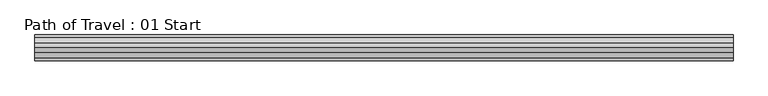
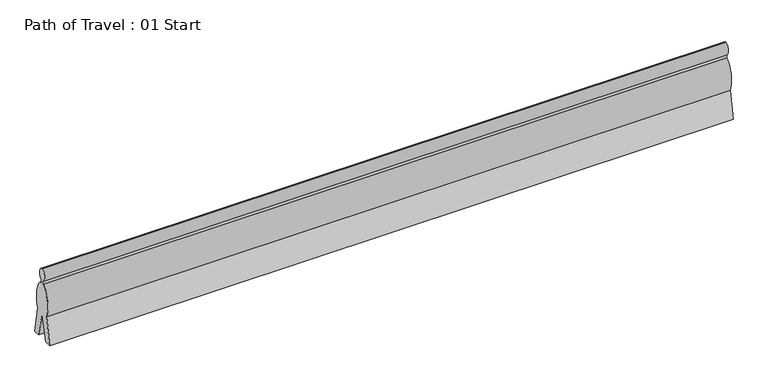
"""IFC4 building model written with IfcOpenShell, lengths in millimetres: proxy geometry, Path of Travel : 01 Start."""

import ifcopenshell
import ifcopenshell.guid

model = None  # the IFC model being written
_history = None  # IfcOwnerHistory: only IFC2X3 demands one
_inside = {}  # id of a spatial element -> (the spatial element, [elements in it])
_under = {}  # id of a project, library or spatial element -> (it, [spatial elements below it])
_declared = {}  # id of a project -> (the project, [libraries it declares])
_typed = {}  # id of a type object -> (the type object, [elements of that type])
_made_of = {}  # id of a material, layer set ... -> (it, [elements and type objects made of it])


def new_model(schema):
    """Start an empty IFC model of exactly this schema.

    Asked for "IFC4X3", IfcOpenShell would pick the latest addendum, in which some entities
    have other attributes; the version numbers below select the first issue.
    IFC2X3 requires an IfcOwnerHistory on every rooted entity: one is made here for all.
    """
    global model, _history
    if schema == "IFC4X3":
        model = ifcopenshell.file(schema_version=(4, 3, 0, 0))
    else:
        model = ifcopenshell.file(schema=schema)
    _inside.clear()
    _under.clear()
    _declared.clear()
    _typed.clear()
    _made_of.clear()
    _history = None
    if model.schema == "IFC2X3":
        org = make("IfcOrganization", Name="unknown")
        user = make(
            "IfcPersonAndOrganization",
            ThePerson=make("IfcPerson", FamilyName="unknown"),
            TheOrganization=org,
        )
        app = make(
            "IfcApplication",
            ApplicationDeveloper=org,
            Version="unknown",
            ApplicationFullName="unknown",
            ApplicationIdentifier="unknown",
        )
        _history = make(
            "IfcOwnerHistory",
            OwningUser=user,
            OwningApplication=app,
            ChangeAction="ADDED",
            CreationDate=0,
        )
    return model


def make(cls, **values):
    """One entity of the class cls with the attributes given. An attribute that is None is left unset."""
    return model.create_entity(
        cls, **{name: value for name, value in values.items() if value is not None}
    )


def rooted(cls, **values):
    """An entity with a GlobalId (a new one), such as an element, a storey or a relation."""
    return make(cls, GlobalId=ifcopenshell.guid.new(), OwnerHistory=_history, **values)


def si_unit(unit_type, name, prefix=None):
    """IfcSIUnit, for example si_unit("LENGTHUNIT", "METRE", prefix="MILLI")."""
    return make("IfcSIUnit", UnitType=unit_type, Prefix=prefix, Name=name)


def assignment(units):
    """IfcUnitAssignment: the units of a project."""
    return None if units is None else make("IfcUnitAssignment", Units=units)


def point(xyz):
    """IfcCartesianPoint."""
    return None if xyz is None else make("IfcCartesianPoint", Coordinates=xyz)


def direction(xyz):
    """IfcDirection."""
    return None if xyz is None else make("IfcDirection", DirectionRatios=xyz)


def frame(location, z_axis=None, x_axis=None):
    """IfcAxis2Placement3D, a coordinate frame: its origin and axes. An axis left out is left unset."""
    return make(
        "IfcAxis2Placement3D",
        Location=point(location),
        Axis=direction(z_axis),
        RefDirection=direction(x_axis),
    )


def origin():
    """The frame at (0, 0, 0) with its axes left unset."""
    return frame((0.0, 0.0, 0.0))


def place(relative_to, where):
    """IfcLocalPlacement: puts the frame where relative to a parent placement (None: the world)."""
    return make(
        "IfcLocalPlacement", PlacementRelTo=relative_to, RelativePlacement=where
    )


def context(
    kind, dimensions, precision=None, world=None, true_north=None, identifier=None
):
    """IfcGeometricRepresentationContext, for example the 3D "Model" context."""
    return make(
        "IfcGeometricRepresentationContext",
        ContextIdentifier=identifier,
        ContextType=kind,
        CoordinateSpaceDimension=dimensions,
        Precision=precision,
        WorldCoordinateSystem=world,
        TrueNorth=true_north,
    )


def project(units=None, contexts=None):
    """IfcProject with its units and contexts."""
    return rooted(
        "IfcProject",
        Name="project",
        RepresentationContexts=contexts,
        UnitsInContext=assignment(units),
    )


def spatial(cls, under=None, at=None, **own):
    """A site, building, storey or space (cls), placed at a placement, below another one or the project."""
    s = rooted(cls, ObjectPlacement=at, **own)
    if under is not None:
        _under.setdefault(under.id(), (under, []))[1].append(s)
    return s


def ellipse_curve(where, semi_axis1, semi_axis2):
    """IfcEllipse in the frame where."""
    return make(
        "IfcEllipse", Position=where, SemiAxis1=semi_axis1, SemiAxis2=semi_axis2
    )


def trimmed(basis, trim1, trim2, sense, master):
    """IfcTrimmedCurve: the piece of a basis curve between two trims."""
    return make(
        "IfcTrimmedCurve",
        BasisCurve=basis,
        Trim1=trim1,
        Trim2=trim2,
        SenseAgreement=sense,
        MasterRepresentation=master,
    )


def shape(context_of_items, identifier, shape_type, items):
    """IfcShapeRepresentation: the items that make up one representation, for example the "Body"."""
    return make(
        "IfcShapeRepresentation",
        ContextOfItems=context_of_items,
        RepresentationIdentifier=identifier,
        RepresentationType=shape_type,
        Items=items,
    )


def source(mapping_origin, context_of_items, identifier, shape_type, items):
    """IfcRepresentationMap: a shape defined once, which mapped items show again and again."""
    return make(
        "IfcRepresentationMap",
        MappingOrigin=mapping_origin,
        MappedRepresentation=shape(context_of_items, identifier, shape_type, items),
    )


def transform(
    local_origin,
    x_axis=None,
    y_axis=None,
    z_axis=None,
    scale=None,
    scale2=None,
    scale3=None,
    uniform=True,
):
    """IfcCartesianTransformationOperator3D, or its non-uniform kind. x_axis, y_axis, z_axis: its Axis1, 2, 3."""
    if uniform:
        return make(
            "IfcCartesianTransformationOperator3D",
            Axis1=direction(x_axis),
            Axis2=direction(y_axis),
            LocalOrigin=point(local_origin),
            Scale=scale,
            Axis3=direction(z_axis),
        )
    return make(
        "IfcCartesianTransformationOperator3DnonUniform",
        Axis1=direction(x_axis),
        Axis2=direction(y_axis),
        LocalOrigin=point(local_origin),
        Scale=scale,
        Axis3=direction(z_axis),
        Scale2=scale2,
        Scale3=scale3,
    )


def mapped(mapping_source, mapping_target):
    """IfcMappedItem: shows the shape of a source again, moved by a transform."""
    return make(
        "IfcMappedItem", MappingSource=mapping_source, MappingTarget=mapping_target
    )


def made_of(thing, what):
    """Note that an element or type object is made of a material, layer set ...; save() writes the relation."""
    if what is not None:
        _made_of.setdefault(what.id(), (what, []))[1].append(thing)
    return thing


def element(
    cls,
    number,
    at=None,
    inside=None,
    cuts=None,
    type_object=None,
    material=None,
    context=None,
    identifier="Body",
    shape_type=None,
    held_by="IfcProductDefinitionShape",
    body=None,
    shapes=None,
    **own,
):
    """One element of the class cls, such as IfcWall. Its Tag is "e" and its number.

    at: its placement. inside: the storey or other place that contains it. cuts: it is an
    opening in that element (IfcRelVoidsElement). A single representation is given by context,
    identifier, shape_type and body (its items); several are given by shapes. held_by: the class
    of the entity that holds the representations. save() writes the other relations.
    """
    e = rooted(cls, Tag="e%d" % number, ObjectPlacement=at, **own)
    if body is not None:
        shapes = [shape(context, identifier, shape_type, body)]
    if shapes is not None:
        e.Representation = make(held_by, Representations=shapes)
    if inside is not None:
        _inside.setdefault(inside.id(), (inside, []))[1].append(e)
    if cuts is not None:
        rooted(
            "IfcRelVoidsElement", RelatingBuildingElement=cuts, RelatedOpeningElement=e
        )
    if type_object is not None:
        _typed.setdefault(type_object.id(), (type_object, []))[1].append(e)
    return made_of(e, material)


def aggregate(whole, parts):
    """IfcRelAggregates: a whole, such as a stair, and the parts it consists of."""
    return rooted("IfcRelAggregates", RelatingObject=whole, RelatedObjects=parts)


def save(model, path):
    """Write the relations noted so far, then the file.

    IfcRelAggregates (storeys below a building ...), IfcRelContainedInSpatialStructure (elements
    in a storey), IfcRelDefinesByType, IfcRelAssociatesMaterial and IfcRelDeclares: one each for
    every whole, place, type object, material and project.
    """
    for whole, parts in _under.values():
        aggregate(whole, parts)
    for where, things in _inside.values():
        rooted(
            "IfcRelContainedInSpatialStructure",
            RelatedElements=things,
            RelatingStructure=where,
        )
    for kind, things in _typed.values():
        rooted("IfcRelDefinesByType", RelatedObjects=things, RelatingType=kind)
    for what, things in _made_of.values():
        rooted("IfcRelAssociatesMaterial", RelatedObjects=things, RelatingMaterial=what)
    for by, libraries in _declared.values():
        rooted("IfcRelDeclares", RelatingContext=by, RelatedDefinitions=libraries)
    model.write(path)


def plane_surface(at):
    """IfcPlane: the flat surface through the origin of the frame at, square to its z axis."""
    return make("IfcPlane", Position=at)


def extruded_surface(curve, direction_of_extrusion, depth):
    """IfcSurfaceOfLinearExtrusion: the curve pushed along a direction by depth."""
    return make(
        "IfcSurfaceOfLinearExtrusion",
        SweptCurve=make("IfcArbitraryOpenProfileDef", ProfileType="CURVE", Curve=curve),
        ExtrudedDirection=direction(direction_of_extrusion),
        Depth=depth,
    )


def advanced_brep(points, edges, surfaces, faces):
    """IfcAdvancedBrep: a solid bounded by faces that lie on surfaces and meet in shared edges.

    An edge is (start, end): straight between two places in points (the first is 0);
    or (start, end, curve); or (start, end, curve, False) where it runs against its curve.
    A face is (place in surfaces, loops), or (place, loops, False) where it looks against
    its surface's normal. A loop lists edges by number (the first is 1), with a minus sign
    where the edge is run from its end to its start. The first loop is the outer one.
    """
    corners = [point(p) for p in points]
    vertices = [make("IfcVertexPoint", VertexGeometry=c) for c in corners]
    made = []
    for start, end, *more in edges:
        made.append(
            make(
                "IfcEdgeCurve",
                EdgeStart=vertices[start],
                EdgeEnd=vertices[end],
                EdgeGeometry=more[0] if more else make("IfcPolyline", Points=[corners[start], corners[end]]),
                SameSense=more[1] if len(more) > 1 else True,
            )
        )
    hull = []
    for where, loops, *sense in faces:
        bounds = []
        for j, loop in enumerate(loops):
            ring = [make("IfcOrientedEdge", EdgeElement=made[abs(k) - 1], Orientation=k > 0) for k in loop]
            bounds.append(
                make(
                    "IfcFaceOuterBound" if j == 0 else "IfcFaceBound",
                    Bound=make("IfcEdgeLoop", EdgeList=ring),
                    Orientation=True,
                )
            )
        hull.append(make("IfcAdvancedFace", Bounds=bounds, FaceSurface=surfaces[where], SameSense=sense[0] if sense else True))
    return make("IfcAdvancedBrep", Outer=make("IfcClosedShell", CfsFaces=hull))


def path_of_travel_01_start_60fd2745(model_context):
    return source(origin(), model_context, "Body", "AdvancedBrep", [
        advanced_brep(
        [(227.5554837, 0.0, 1727.2), (227.5554837, 42.9018657, 1436.6534209), (227.5554837, 42.9018657, 1363.4763406), (227.5554837, 184.1186263, 643.4144547), (227.5554837, 297.5699544, 0.0), (227.5554837, 145.6574193, 0.0), (227.5554837, 0.0, 584.2), (227.5554837, -145.6574193, 0.0), (227.5554837, -297.5699544, 0.0), (227.5554837, -184.1186263, 643.4144547), (227.5554837, -42.9018657, 1363.4763406), (227.5554837, -42.9018657, 1436.6534209), (16229.5554837, 0.0, 1727.2), (16229.5554837, -42.9018657, 1436.6534209), (16229.5554837, -42.9018657, 1363.4763406), (16229.5554837, -184.1186263, 643.4144547), (16229.5554837, -297.5699544, 0.0), (16229.5554837, -145.6574193, 0.0), (16229.5554837, 0.0, 584.2), (16229.5554837, 145.6574193, 0.0), (16229.5554837, 297.5699544, 0.0), (16229.5554837, 184.1186263, 643.4144547), (16229.5554837, 42.9018657, 1363.4763406), (16229.5554837, 42.9018657, 1436.6534209)],
        [
            (0, 1, ellipse_curve(frame((227.5554837, 0.0, 1574.8), z_axis=(-1.0, 0.0, 0.0), x_axis=(0.0, 0.0, 1.0)), 152.4, 101.6)),
            (1, 2),
            (2, 3, ellipse_curve(frame((227.5554837, 0.0, 914.4), z_axis=(-1.0, 0.0, 0.0), x_axis=(0.0, 0.0, -1.0)), 457.2, 228.6)),
            (3, 4),
            (4, 5),
            (5, 6),
            (6, 7),
            (7, 8),
            (8, 9),
            (9, 10, ellipse_curve(frame((227.5554837, 0.0, 914.4), z_axis=(-1.0, 0.0, 0.0), x_axis=(0.0, 0.0, -1.0)), 457.2, 228.6)),
            (10, 11),
            (11, 0, ellipse_curve(frame((227.5554837, 0.0, 1574.8), z_axis=(-1.0, 0.0, 0.0), x_axis=(0.0, 0.0, 1.0)), 152.4, 101.6)),
            (12, 13, ellipse_curve(frame((16229.5554837, 0.0, 1574.8), z_axis=(1.0, 0.0, 0.0), x_axis=(0.0, 0.0, 1.0)), 152.4, 101.6)),
            (13, 14),
            (14, 15, ellipse_curve(frame((16229.5554837, 0.0, 914.4), z_axis=(1.0, 0.0, 0.0), x_axis=(0.0, 0.0, -1.0)), 457.2, 228.6)),
            (15, 16),
            (16, 17),
            (17, 18),
            (18, 19),
            (19, 20),
            (20, 21),
            (21, 22, ellipse_curve(frame((16229.5554837, 0.0, 914.4), z_axis=(1.0, 0.0, 0.0), x_axis=(0.0, 0.0, -1.0)), 457.2, 228.6)),
            (22, 23),
            (23, 12, ellipse_curve(frame((16229.5554837, 0.0, 1574.8), z_axis=(1.0, 0.0, 0.0), x_axis=(0.0, 0.0, 1.0)), 152.4, 101.6)),
            (0, 12),
            (23, 1),
            (22, 2),
            (21, 3),
            (20, 4),
            (19, 5),
            (18, 6),
            (17, 7),
            (16, 8),
            (15, 9),
            (14, 10),
            (13, 11),
        ],
        [
            plane_surface(frame((227.5554837, 0.0, 0.0), z_axis=(-1.0, 0.0, 0.0), x_axis=(0.0, 0.0, 1.0))),
            plane_surface(frame((16229.5554837, 0.0, 0.0), z_axis=(1.0, 0.0, 0.0), x_axis=(0.0, 0.0, 1.0))),
            extruded_surface(trimmed(ellipse_curve(frame((16229.5554837, 0.0, 1574.8), z_axis=(-1.0, 0.0, 0.0), x_axis=(0.0, 0.0, 1.0)), 152.4, 101.6), [point((16229.5554837, 0.0, 1727.2))], [point((16229.5554837, 42.9018657, 1436.6534209))], True, "CARTESIAN"), (-16002.0, 0.0, 0.0), 16002.0),
            plane_surface(frame((227.5554837, 42.9018657, 1436.6534209), z_axis=(0.0, 1.0, 0.0), x_axis=(1.0, 0.0, 0.0))),
            extruded_surface(trimmed(ellipse_curve(frame((16229.5554837, 0.0, 914.4), z_axis=(-1.0, 0.0, 0.0), x_axis=(0.0, 0.0, -1.0)), 457.2, 228.6), [point((16229.5554837, 42.9018657, 1363.4763406))], [point((16229.5554837, 184.1186263, 643.4144547))], True, "CARTESIAN"), (-16002.0, 0.0, 0.0), 16002.0),
            plane_surface(frame((227.5554837, 184.1186263, 643.4144547), z_axis=(0.0, 0.9848077530122078, 0.17364817766693205), x_axis=(1.0, 0.0, 0.0))),
            plane_surface(frame((227.5554837, 297.5699544, 0.0), z_axis=(0.0, 0.0, -1.0), x_axis=(1.0, 0.0, 0.0))),
            plane_surface(frame((227.5554837, 145.6574193, 0.0), z_axis=(0.0, -0.9702957262760199, -0.2419218955995739), x_axis=(1.0, 0.0, 0.0))),
            plane_surface(frame((227.5554837, 0.0, 584.2), z_axis=(0.0, 0.9702957262759961, -0.24192189559966923), x_axis=(1.0, 0.0, 0.0))),
            plane_surface(frame((227.5554837, -145.6574193, 0.0), z_axis=(0.0, 0.0, -1.0), x_axis=(1.0, 0.0, 0.0))),
            plane_surface(frame((227.5554837, -297.5699544, 0.0), z_axis=(0.0, -0.984807753012208, 0.17364817766693066), x_axis=(1.0, 0.0, 0.0))),
            extruded_surface(trimmed(ellipse_curve(frame((16229.5554837, 0.0, 914.4), z_axis=(-1.0, 0.0, 0.0), x_axis=(0.0, 0.0, -1.0)), 457.2, 228.6), [point((16229.5554837, -184.1186263, 643.4144547))], [point((16229.5554837, -42.9018657, 1363.4763406))], True, "CARTESIAN"), (-16002.0, 0.0, 0.0), 16002.0),
            plane_surface(frame((227.5554837, -42.9018657, 1363.4763406), z_axis=(0.0, -1.0, 0.0), x_axis=(1.0, 0.0, 0.0))),
            extruded_surface(trimmed(ellipse_curve(frame((16229.5554837, 0.0, 1574.8), z_axis=(-1.0, 0.0, 0.0), x_axis=(0.0, 0.0, 1.0)), 152.4, 101.6), [point((16229.5554837, -42.9018657, 1436.6534209))], [point((16229.5554837, 0.0, 1727.2))], True, "CARTESIAN"), (-16002.0, 0.0, 0.0), 16002.0),
        ],
        [
            (0, [[1, 2, 3, 4, 5, 6, 7, 8, 9, 10, 11, 12]]),
            (1, [[13, 14, 15, 16, 17, 18, 19, 20, 21, 22, 23, 24]]),
            (2, [[-1, 25, -24, 26]]),
            (3, [[-2, -26, -23, 27]]),
            (4, [[-3, -27, -22, 28]]),
            (5, [[-4, -28, -21, 29]]),
            (6, [[-5, -29, -20, 30]]),
            (7, [[-6, -30, -19, 31]]),
            (8, [[-7, -31, -18, 32]]),
            (9, [[-8, -32, -17, 33]]),
            (10, [[-9, -33, -16, 34]]),
            (11, [[-10, -34, -15, 35]]),
            (12, [[-11, -35, -14, 36]]),
            (13, [[-12, -36, -13, -25]]),
        ],
    ),
    ])


if __name__ == "__main__":
    model = new_model("IFC4")
    model_context = context("Model", 3, world=origin())
    ifc_project = project(units=[si_unit("LENGTHUNIT", "METRE", prefix="MILLI")], contexts=[model_context])
    site = spatial("IfcSite", under=ifc_project)
    building = spatial("IfcBuilding", under=site)
    placement = place(None, origin())
    path_of_travel_01_start_shape = path_of_travel_01_start_60fd2745(model_context)
    element("IfcBuildingElementProxy", 1, Name="Path of Travel : 01 Start", ObjectType="Path of Travel : 01 Start", at=placement, inside=building, context=model_context, shape_type="MappedRepresentation", body=[
        mapped(path_of_travel_01_start_shape, transform((0.0, 0.0, 0.0), x_axis=(1.0, 0.0, 0.0), y_axis=(0.0, 1.0, 0.0), z_axis=(0.0, 0.0, 1.0))),
    ])
    save(model, "model.ifc")

# Revit data of these elements
# Type "Path of Travel : 01 Start"
#   Path of Egress [instance default] = 4' - 0"
#   built-in parameter 1001306 [instance default] = 4 (stored number, unit not read)
#   Dot at Start = yes
#   Arrow in Middle = yes
#   Arrow at End = no
#   Egress Path = none
# Element 1 (IfcBuildingElementProxy, "Path of Travel : 01 Start")
#   Path of Egress = 52' - 6"
#   built-in parameter 1001306 = 52.5 (stored number, unit not read)
#   Materials on its faces: "Egress Path Solid"
# Materials
#   "Egress Path Solid": class "Unassigned", colour RGB 255 128 64, transparency 0.75, Comments = "Rendering appearance not upgraded "
